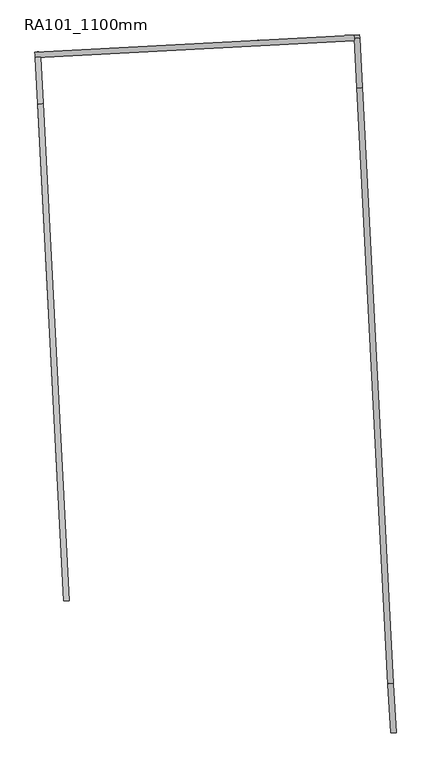
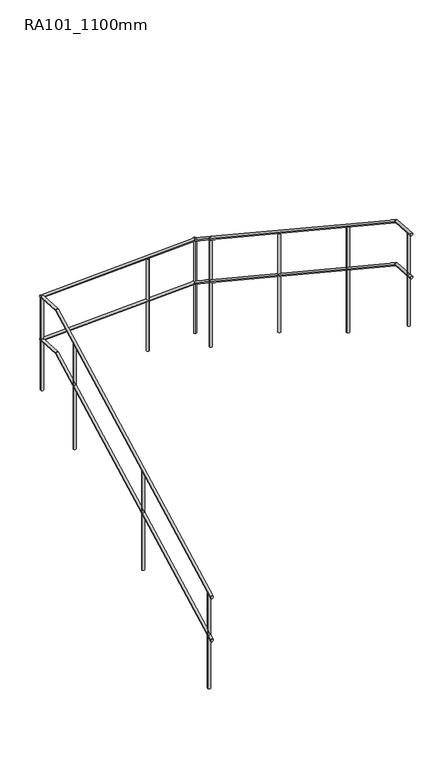
"""IFC4 building model written with IfcOpenShell, lengths in millimetres: railing geometry, RA101_1100mm."""

from ifc_helpers import new_model, si_unit, point, frame, frame_2d, origin, place, context, project, spatial, circle_curve, ellipse_curve, trimmed, segment, composite_curve, outline, extrude, source, transform, mapped, element, save
from ifc_brep_helpers import plane_surface, cylinder_surface, advanced_brep


def ra101_1100mm_54c19647(model_context):
    return source(origin(), model_context, "Body", "SolidModel", [
        advanced_brep(
        [(22896.1789103, 12534.7141331, 457.1248327), (22926.1377964, 12536.2842117, 457.1248327), (22754.6396676, 15235.4437699, 2210.0), (22784.5985536, 15237.0138486, 2210.0), (22741.5052252, 15486.0638601, 2210.0), (22771.4641113, 15487.6339388, 2210.0)],
        [
            (0, 1, ellipse_curve(frame((22911.1583533, 12535.4991724, 457.1248327), z_axis=(0.05233595624294174, -0.998629534754574, 0.0), x_axis=(0.0, 0.0, -0.9999999999999999)), 17.8751673, 15.0)),
            (1, 0, ellipse_curve(frame((22911.1583533, 12535.4991724, 457.1248327), z_axis=(0.05233595624294174, -0.998629534754574, 0.0), x_axis=(0.0, 0.0, -0.9999999999999999)), 17.8751673, 15.0)),
            (0, 2),
            (2, 3, ellipse_curve(frame((22769.6191106, 15236.2288092, 2210.0), z_axis=(0.05018733030882238, -0.9576313096148807, -0.28359038545367066), x_axis=(-0.014841974004015643, 0.28320173468646914, -0.9589455111101144)), 15.6421818, 15.0)),
            (3, 1),
            (3, 2, ellipse_curve(frame((22769.6191106, 15236.2288092, 2210.0), z_axis=(0.05018733030882238, -0.9576313096148807, -0.28359038545367066), x_axis=(-0.014841974004015643, 0.28320173468646914, -0.9589455111101144)), 15.6421818, 15.0)),
            (4, 5, circle_curve(frame((22756.4846683, 15486.8488994, 2210.0), z_axis=(-0.05233595624293797, 0.9986295347545743, 0.0), x_axis=(0.9986295347545743, 0.05233595624293797, 0.0)), 15.0)),
            (5, 4, circle_curve(frame((22756.4846683, 15486.8488994, 2210.0), z_axis=(-0.05233595624293797, 0.9986295347545743, 0.0), x_axis=(0.9986295347545743, 0.05233595624293797, 0.0)), 15.0)),
            (2, 4),
            (5, 3),
        ],
        [
            plane_surface(frame((22911.1583533, 12535.4991724, 475.0), z_axis=(0.05233595624294174, -0.998629534754574, 0.0), x_axis=(0.998629534754574, 0.05233595624294174, 0.0))),
            cylinder_surface(frame((22910.731374, 12543.6464234, 462.4127052), z_axis=(0.04391787398555367, -0.8380029565528062, -0.5438954542495689), x_axis=(0.998629534754574, 0.052335956242941746, 0.0)), 15.0),
            plane_surface(frame((22756.4846683, 15486.8488994, 2225.0), z_axis=(-0.05233595624294184, 0.998629534754574, 0.0), x_axis=(0.998629534754574, 0.05233595624294184, 0.0))),
            cylinder_surface(frame((22769.8512715, 15231.7989162, 2210.0), z_axis=(0.05233595624293797, -0.9986295347545743, 0.0), x_axis=(0.9986295347545743, 0.05233595624293797, 0.0)), 15.0),
        ],
        [
            (0, [[1, 2]]),
            (1, [[-1, 3, 4, 5]]),
            (1, [[-2, -5, 6, -3]]),
            (2, [[7, 8]]),
            (3, [[-4, 9, -8, 10]]),
            (3, [[-6, -10, -7, -9]]),
        ],
    ),
        advanced_brep(
        [(22739.9351465, 15516.0227461, 2210.0), (22741.5052252, 15486.0638601, 2210.0), (24475.8528668, 15606.9983388, 2210.0), (24477.4229455, 15577.0394528, 2210.0)],
        [
            (0, 1, circle_curve(frame((22740.7201859, 15501.0433031, 2210.0), z_axis=(-0.998629534754574, -0.05233595624294185, 0.0), x_axis=(0.05233595624294185, -0.998629534754574, 0.0)), 15.0)),
            (1, 0, circle_curve(frame((22740.7201859, 15501.0433031, 2210.0), z_axis=(-0.998629534754574, -0.05233595624294185, 0.0), x_axis=(0.05233595624294185, -0.998629534754574, 0.0)), 15.0)),
            (2, 3, circle_curve(frame((24476.6379061, 15592.0188958, 2210.0), z_axis=(0.998629534754574, 0.05233595624294185, 0.0), x_axis=(0.05233595624294185, -0.998629534754574, 0.0)), 15.0)),
            (3, 2, circle_curve(frame((24476.6379061, 15592.0188958, 2210.0), z_axis=(0.998629534754574, 0.05233595624294185, 0.0), x_axis=(0.05233595624294185, -0.998629534754574, 0.0)), 15.0)),
            (0, 2),
            (3, 1),
        ],
        [
            plane_surface(frame((22740.7201859, 15501.0433031, 2225.0), z_axis=(-0.9986295347545743, -0.052335956242937944, 0.0), x_axis=(0.052335956242937944, -0.9986295347545743, 0.0))),
            plane_surface(frame((24476.6379061, 15592.0188958, 2225.0), z_axis=(0.9986295347545743, 0.052335956242937104, 0.0), x_axis=(0.052335956242937104, -0.9986295347545743, 0.0))),
            cylinder_surface(frame((22740.7201859, 15501.0433031, 2210.0), z_axis=(-0.998629534754574, -0.05233595624294185, 0.0), x_axis=(0.05233595624294185, -0.998629534754574, 0.0)), 15.0),
        ],
        [
            (0, [[1, 2]]),
            (1, [[3, 4]]),
            (2, [[-1, 5, -4, 6]]),
            (2, [[-2, -6, -3, -5]]),
        ],
    ),
        advanced_brep(
        [(24505.8117528, 15608.5684175, 2210.0), (24475.8528668, 15606.9983388, 2210.0), (24506.8498874, 15588.7596297, 2210.0), (24476.8910014, 15587.189551, 2210.0), (24520.7484348, 15323.5595483, 2382.1248327), (24490.7895487, 15321.9894696, 2382.1248327)],
        [
            (0, 1, circle_curve(frame((24490.8323098, 15607.7833782, 2210.0), z_axis=(-0.052335956242937104, 0.9986295347545743, 0.0), x_axis=(-0.9986295347545743, -0.052335956242937104, 0.0)), 15.0)),
            (1, 0, circle_curve(frame((24490.8323098, 15607.7833782, 2210.0), z_axis=(-0.052335956242937104, 0.9986295347545743, 0.0), x_axis=(-0.9986295347545743, -0.052335956242937104, 0.0)), 15.0)),
            (0, 2),
            (2, 3, ellipse_curve(frame((24491.8704444, 15587.9745903, 2210.0), z_axis=(-0.050187330308819895, 0.9576313096148807, -0.28359038545367116), x_axis=(-0.014841974004020982, 0.2832017346864703, 0.9589455111101142)), 15.6421818, 15.0)),
            (3, 1),
            (3, 2, ellipse_curve(frame((24491.8704444, 15587.9745903, 2210.0), z_axis=(-0.050187330308819895, 0.9576313096148807, -0.28359038545367116), x_axis=(-0.014841974004020982, 0.2832017346864703, 0.9589455111101142)), 15.6421818, 15.0)),
            (4, 5, ellipse_curve(frame((24505.7689917, 15322.774509, 2382.1248327), z_axis=(0.052335956242937104, -0.9986295347545743, 0.0), x_axis=(0.0, 0.0, -1.0)), 17.8751673, 15.0)),
            (5, 4, ellipse_curve(frame((24505.7689917, 15322.774509, 2382.1248327), z_axis=(0.052335956242937104, -0.9986295347545743, 0.0), x_axis=(0.0, 0.0, -1.0)), 17.8751673, 15.0)),
            (2, 4),
            (5, 3),
        ],
        [
            plane_surface(frame((24490.8323098, 15607.7833782, 2225.0), z_axis=(-0.05233595624294184, 0.998629534754574, 0.0), x_axis=(0.998629534754574, 0.05233595624294184, 0.0))),
            cylinder_surface(frame((24490.8323098, 15607.7833782, 2210.0), z_axis=(-0.052335956242937104, 0.9986295347545743, 0.0), x_axis=(-0.9986295347545743, -0.052335956242937104, 0.0)), 15.0),
            plane_surface(frame((24505.7689917, 15322.774509, 2400.0), z_axis=(0.052335956242937104, -0.9986295347545743, 0.0), x_axis=(0.9986295347545743, 0.052335956242937104, 0.0))),
            cylinder_surface(frame((24492.0652629, 15584.2572324, 2212.4127052), z_axis=(-0.04391787398554974, 0.8380029565528057, -0.5438954542495701), x_axis=(-0.9986295347545743, -0.0523359562429371, 0.0)), 15.0),
        ],
        [
            (0, [[1, 2]]),
            (1, [[-1, 3, 4, 5]]),
            (1, [[-2, -5, 6, -3]]),
            (2, [[7, 8]]),
            (3, [[-4, 9, -8, 10]]),
            (3, [[-6, -10, -7, -9]]),
        ],
    ),
        advanced_brep(
        [(24520.7484348, 15323.5595483, 2382.1248327), (24490.7895487, 15321.9894696, 2382.1248327), (24690.5490938, 12083.5699627, 4485.0), (24660.5902078, 12081.999884, 4485.0), (24704.4476412, 11818.3698813, 4485.0), (24674.4887551, 11816.7998026, 4485.0)],
        [
            (0, 1, ellipse_curve(frame((24505.7689917, 15322.774509, 2382.1248327), z_axis=(-0.05233595624294191, 0.998629534754574, 0.0), x_axis=(0.0, 0.0, -1.0)), 17.8751673, 15.0)),
            (1, 0, ellipse_curve(frame((24505.7689917, 15322.774509, 2382.1248327), z_axis=(-0.05233595624294191, 0.998629534754574, 0.0), x_axis=(0.0, 0.0, -1.0)), 17.8751673, 15.0)),
            (0, 2),
            (2, 3, ellipse_curve(frame((24675.5696508, 12082.7849234, 4485.0), z_axis=(-0.05018733030882025, 0.9576313096148807, -0.28359038545367127), x_axis=(0.014841974004007963, -0.28320173468647103, -0.9589455111101143)), 15.6421818, 15.0)),
            (3, 1),
            (3, 2, ellipse_curve(frame((24675.5696508, 12082.7849234, 4485.0), z_axis=(-0.05018733030882025, 0.9576313096148807, -0.28359038545367127), x_axis=(0.014841974004007963, -0.28320173468647103, -0.9589455111101143)), 15.6421818, 15.0)),
            (4, 5, circle_curve(frame((24689.4681982, 11817.584842, 4485.0), z_axis=(0.05233595624293375, -0.9986295347545745, 0.0), x_axis=(-0.9986295347545745, -0.05233595624293375, 0.0)), 15.0)),
            (5, 4, circle_curve(frame((24689.4681982, 11817.584842, 4485.0), z_axis=(0.05233595624293375, -0.9986295347545745, 0.0), x_axis=(-0.9986295347545745, -0.05233595624293375, 0.0)), 15.0)),
            (2, 4),
            (5, 3),
        ],
        [
            plane_surface(frame((24505.7689917, 15322.774509, 2400.0), z_axis=(-0.05233595624294191, 0.998629534754574, 0.0), x_axis=(0.998629534754574, 0.05233595624294191, 0.0))),
            cylinder_surface(frame((24506.1959711, 15314.627258, 2387.4127052), z_axis=(-0.04391787398555378, 0.8380029565528053, -0.5438954542495702), x_axis=(-0.998629534754574, -0.052335956242941926, 0.0)), 15.0),
            plane_surface(frame((24689.4681982, 11817.584842, 4500.0), z_axis=(0.05233595624293375, -0.9986295347545745, 0.0), x_axis=(0.9986295347545745, 0.05233595624293375, 0.0))),
            cylinder_surface(frame((24675.33749, 12087.2148164, 4485.0), z_axis=(-0.05233595624293375, 0.9986295347545745, 0.0), x_axis=(-0.9986295347545745, -0.05233595624293375, 0.0)), 15.0),
        ],
        [
            (0, [[1, 2]]),
            (1, [[-1, 3, 4, 5]]),
            (1, [[-2, -5, 6, -3]]),
            (2, [[7, 8]]),
            (3, [[-4, 9, -8, 10]]),
            (3, [[-6, -10, -7, -9]]),
        ],
    ),
        advanced_brep(
        [(22896.1789103, 12534.7141331, 957.1248327), (22926.1377964, 12536.2842117, 957.1248327), (22754.6396676, 15235.4437699, 2710.0), (22784.5985536, 15237.0138486, 2710.0), (22741.5052252, 15486.0638601, 2710.0), (22771.4641113, 15487.6339388, 2710.0)],
        [
            (0, 1, ellipse_curve(frame((22911.1583533, 12535.4991724, 957.1248327), z_axis=(0.05233595624294174, -0.998629534754574, 0.0), x_axis=(0.0, 0.0, -0.9999999999999999)), 17.8751673, 15.0)),
            (1, 0, ellipse_curve(frame((22911.1583533, 12535.4991724, 957.1248327), z_axis=(0.05233595624294174, -0.998629534754574, 0.0), x_axis=(0.0, 0.0, -0.9999999999999999)), 17.8751673, 15.0)),
            (0, 2),
            (2, 3, ellipse_curve(frame((22769.6191106, 15236.2288092, 2710.0), z_axis=(0.05018733030882238, -0.9576313096148807, -0.28359038545367066), x_axis=(-0.014841974004015643, 0.28320173468646914, -0.9589455111101144)), 15.6421818, 15.0)),
            (3, 1),
            (3, 2, ellipse_curve(frame((22769.6191106, 15236.2288092, 2710.0), z_axis=(0.05018733030882238, -0.9576313096148807, -0.28359038545367066), x_axis=(-0.014841974004015643, 0.28320173468646914, -0.9589455111101144)), 15.6421818, 15.0)),
            (4, 5, circle_curve(frame((22756.4846683, 15486.8488994, 2710.0), z_axis=(-0.05233595624293797, 0.9986295347545743, 0.0), x_axis=(0.9986295347545743, 0.05233595624293797, 0.0)), 15.0)),
            (5, 4, circle_curve(frame((22756.4846683, 15486.8488994, 2710.0), z_axis=(-0.05233595624293797, 0.9986295347545743, 0.0), x_axis=(0.9986295347545743, 0.05233595624293797, 0.0)), 15.0)),
            (2, 4),
            (5, 3),
        ],
        [
            plane_surface(frame((22911.1583533, 12535.4991724, 975.0), z_axis=(0.05233595624294174, -0.998629534754574, 0.0), x_axis=(0.998629534754574, 0.05233595624294174, 0.0))),
            cylinder_surface(frame((22910.731374, 12543.6464234, 962.4127052), z_axis=(0.04391787398555367, -0.8380029565528062, -0.5438954542495689), x_axis=(0.998629534754574, 0.052335956242941746, 0.0)), 15.0),
            plane_surface(frame((22756.4846683, 15486.8488994, 2725.0), z_axis=(-0.05233595624294184, 0.998629534754574, 0.0), x_axis=(0.998629534754574, 0.05233595624294184, 0.0))),
            cylinder_surface(frame((22769.8512715, 15231.7989162, 2710.0), z_axis=(0.05233595624293797, -0.9986295347545743, 0.0), x_axis=(0.9986295347545743, 0.05233595624293797, 0.0)), 15.0),
        ],
        [
            (0, [[1, 2]]),
            (1, [[-1, 3, 4, 5]]),
            (1, [[-2, -5, 6, -3]]),
            (2, [[7, 8]]),
            (3, [[-4, 9, -8, 10]]),
            (3, [[-6, -10, -7, -9]]),
        ],
    ),
        advanced_brep(
        [(22739.9351465, 15516.0227461, 2710.0), (22741.5052252, 15486.0638601, 2710.0), (24475.8528668, 15606.9983388, 2710.0), (24477.4229455, 15577.0394528, 2710.0)],
        [
            (0, 1, circle_curve(frame((22740.7201859, 15501.0433031, 2710.0), z_axis=(-0.998629534754574, -0.05233595624294185, 0.0), x_axis=(0.05233595624294185, -0.998629534754574, 0.0)), 15.0)),
            (1, 0, circle_curve(frame((22740.7201859, 15501.0433031, 2710.0), z_axis=(-0.998629534754574, -0.05233595624294185, 0.0), x_axis=(0.05233595624294185, -0.998629534754574, 0.0)), 15.0)),
            (2, 3, circle_curve(frame((24476.6379061, 15592.0188958, 2710.0), z_axis=(0.998629534754574, 0.05233595624294185, 0.0), x_axis=(0.05233595624294185, -0.998629534754574, 0.0)), 15.0)),
            (3, 2, circle_curve(frame((24476.6379061, 15592.0188958, 2710.0), z_axis=(0.998629534754574, 0.05233595624294185, 0.0), x_axis=(0.05233595624294185, -0.998629534754574, 0.0)), 15.0)),
            (0, 2),
            (3, 1),
        ],
        [
            plane_surface(frame((22740.7201859, 15501.0433031, 2725.0), z_axis=(-0.9986295347545743, -0.052335956242937944, 0.0), x_axis=(0.052335956242937944, -0.9986295347545743, 0.0))),
            plane_surface(frame((24476.6379061, 15592.0188958, 2725.0), z_axis=(0.9986295347545743, 0.052335956242937104, 0.0), x_axis=(0.052335956242937104, -0.9986295347545743, 0.0))),
            cylinder_surface(frame((22740.7201859, 15501.0433031, 2710.0), z_axis=(-0.998629534754574, -0.05233595624294185, 0.0), x_axis=(0.05233595624294185, -0.998629534754574, 0.0)), 15.0),
        ],
        [
            (0, [[1, 2]]),
            (1, [[3, 4]]),
            (2, [[-1, 5, -4, 6]]),
            (2, [[-2, -6, -3, -5]]),
        ],
    ),
        advanced_brep(
        [(24505.8117528, 15608.5684175, 2710.0), (24475.8528668, 15606.9983388, 2710.0), (24506.8498874, 15588.7596297, 2710.0), (24476.8910014, 15587.189551, 2710.0), (24520.7484348, 15323.5595483, 2882.1248327), (24490.7895487, 15321.9894696, 2882.1248327)],
        [
            (0, 1, circle_curve(frame((24490.8323098, 15607.7833782, 2710.0), z_axis=(-0.052335956242937104, 0.9986295347545743, 0.0), x_axis=(-0.9986295347545743, -0.052335956242937104, 0.0)), 15.0)),
            (1, 0, circle_curve(frame((24490.8323098, 15607.7833782, 2710.0), z_axis=(-0.052335956242937104, 0.9986295347545743, 0.0), x_axis=(-0.9986295347545743, -0.052335956242937104, 0.0)), 15.0)),
            (0, 2),
            (2, 3, ellipse_curve(frame((24491.8704444, 15587.9745903, 2710.0), z_axis=(-0.050187330308819895, 0.9576313096148807, -0.28359038545367116), x_axis=(-0.014841974004020982, 0.2832017346864703, 0.9589455111101142)), 15.6421818, 15.0)),
            (3, 1),
            (3, 2, ellipse_curve(frame((24491.8704444, 15587.9745903, 2710.0), z_axis=(-0.050187330308819895, 0.9576313096148807, -0.28359038545367116), x_axis=(-0.014841974004020982, 0.2832017346864703, 0.9589455111101142)), 15.6421818, 15.0)),
            (4, 5, ellipse_curve(frame((24505.7689917, 15322.774509, 2882.1248327), z_axis=(0.052335956242937104, -0.9986295347545743, 0.0), x_axis=(0.0, 0.0, -1.0)), 17.8751673, 15.0)),
            (5, 4, ellipse_curve(frame((24505.7689917, 15322.774509, 2882.1248327), z_axis=(0.052335956242937104, -0.9986295347545743, 0.0), x_axis=(0.0, 0.0, -1.0)), 17.8751673, 15.0)),
            (2, 4),
            (5, 3),
        ],
        [
            plane_surface(frame((24490.8323098, 15607.7833782, 2725.0), z_axis=(-0.05233595624294184, 0.998629534754574, 0.0), x_axis=(0.998629534754574, 0.05233595624294184, 0.0))),
            cylinder_surface(frame((24490.8323098, 15607.7833782, 2710.0), z_axis=(-0.052335956242937104, 0.9986295347545743, 0.0), x_axis=(-0.9986295347545743, -0.052335956242937104, 0.0)), 15.0),
            plane_surface(frame((24505.7689917, 15322.774509, 2900.0), z_axis=(0.052335956242937104, -0.9986295347545743, 0.0), x_axis=(0.9986295347545743, 0.052335956242937104, 0.0))),
            cylinder_surface(frame((24492.0652629, 15584.2572324, 2712.4127052), z_axis=(-0.04391787398554974, 0.8380029565528057, -0.5438954542495701), x_axis=(-0.9986295347545743, -0.0523359562429371, 0.0)), 15.0),
        ],
        [
            (0, [[1, 2]]),
            (1, [[-1, 3, 4, 5]]),
            (1, [[-2, -5, 6, -3]]),
            (2, [[7, 8]]),
            (3, [[-4, 9, -8, 10]]),
            (3, [[-6, -10, -7, -9]]),
        ],
    ),
        advanced_brep(
        [(24520.7484348, 15323.5595483, 2882.1248327), (24490.7895487, 15321.9894696, 2882.1248327), (24690.5490938, 12083.5699627, 4985.0), (24660.5902078, 12081.999884, 4985.0), (24704.4476412, 11818.3698813, 4985.0), (24674.4887551, 11816.7998026, 4985.0)],
        [
            (0, 1, ellipse_curve(frame((24505.7689917, 15322.774509, 2882.1248327), z_axis=(-0.05233595624294191, 0.998629534754574, 0.0), x_axis=(0.0, 0.0, -1.0)), 17.8751673, 15.0)),
            (1, 0, ellipse_curve(frame((24505.7689917, 15322.774509, 2882.1248327), z_axis=(-0.05233595624294191, 0.998629534754574, 0.0), x_axis=(0.0, 0.0, -1.0)), 17.8751673, 15.0)),
            (0, 2),
            (2, 3, ellipse_curve(frame((24675.5696508, 12082.7849234, 4985.0), z_axis=(-0.05018733030882025, 0.9576313096148807, -0.28359038545367127), x_axis=(0.014841974004007963, -0.28320173468647103, -0.9589455111101143)), 15.6421818, 15.0)),
            (3, 1),
            (3, 2, ellipse_curve(frame((24675.5696508, 12082.7849234, 4985.0), z_axis=(-0.05018733030882025, 0.9576313096148807, -0.28359038545367127), x_axis=(0.014841974004007963, -0.28320173468647103, -0.9589455111101143)), 15.6421818, 15.0)),
            (4, 5, circle_curve(frame((24689.4681982, 11817.584842, 4985.0), z_axis=(0.05233595624293375, -0.9986295347545745, 0.0), x_axis=(-0.9986295347545745, -0.05233595624293375, 0.0)), 15.0)),
            (5, 4, circle_curve(frame((24689.4681982, 11817.584842, 4985.0), z_axis=(0.05233595624293375, -0.9986295347545745, 0.0), x_axis=(-0.9986295347545745, -0.05233595624293375, 0.0)), 15.0)),
            (2, 4),
            (5, 3),
        ],
        [
            plane_surface(frame((24505.7689917, 15322.774509, 2900.0), z_axis=(-0.05233595624294191, 0.998629534754574, 0.0), x_axis=(0.998629534754574, 0.05233595624294191, 0.0))),
            cylinder_surface(frame((24506.1959711, 15314.627258, 2887.4127052), z_axis=(-0.04391787398555378, 0.8380029565528053, -0.5438954542495702), x_axis=(-0.998629534754574, -0.052335956242941926, 0.0)), 15.0),
            plane_surface(frame((24689.4681982, 11817.584842, 5000.0), z_axis=(0.05233595624293375, -0.9986295347545745, 0.0), x_axis=(0.9986295347545745, 0.05233595624293375, 0.0))),
            cylinder_surface(frame((24675.33749, 12087.2148164, 4985.0), z_axis=(-0.05233595624293375, 0.9986295347545745, 0.0), x_axis=(-0.9986295347545745, -0.05233595624293375, 0.0)), 15.0),
        ],
        [
            (0, [[1, 2]]),
            (1, [[-1, 3, 4, 5]]),
            (1, [[-2, -5, 6, -3]]),
            (2, [[7, 8]]),
            (3, [[-4, 9, -8, 10]]),
            (3, [[-6, -10, -7, -9]]),
        ],
    ),
        extrude(outline(composite_curve([segment(trimmed(circle_curve(frame_2d((24631.3752867, 12926.0636256)), 15.0), [point((24616.3958437, 12925.2785862))], [point((24646.3547297, 12926.8486649))], False, "CARTESIAN"), True, "CONTINUOUS"), segment(trimmed(circle_curve(frame_2d((24631.3752867, 12926.0636256)), 15.0), [point((24646.3547297, 12926.8486649))], [point((24616.3958437, 12925.2785862))], False, "CARTESIAN"), True, "CONTINUOUS")], self_intersect=False)), frame((0.0, 0.0, 3200.0), z_axis=(0.0, 0.0, 1.0), x_axis=(1.0, 0.0, 0.0)), (0.0, 0.0, 1.0), 1225.5555556),
        extrude(outline(composite_curve([segment(trimmed(circle_curve(frame_2d((24568.5721392, 14124.4190673)), 15.0), [point((24553.5926962, 14123.6340279))], [point((24583.5515823, 14125.2041066))], False, "CARTESIAN"), True, "CONTINUOUS"), segment(trimmed(circle_curve(frame_2d((24568.5721392, 14124.4190673)), 15.0), [point((24583.5515823, 14125.2041066))], [point((24553.5926962, 14123.6340279))], False, "CARTESIAN"), True, "CONTINUOUS")], self_intersect=False)), frame((0.0, 0.0, 2500.0), z_axis=(0.0, 0.0, 1.0), x_axis=(1.0, 0.0, 0.0)), (0.0, 0.0, 1.0), 1147.7777778),
        extrude(outline(composite_curve([segment(trimmed(circle_curve(frame_2d((23954.0550706, 15564.6314899)), 15.0), [point((23954.84011, 15549.6520469))], [point((23953.2700313, 15579.6109329))], False, "CARTESIAN"), True, "CONTINUOUS"), segment(trimmed(circle_curve(frame_2d((23954.0550706, 15564.6314899)), 15.0), [point((23953.2700313, 15579.6109329))], [point((23954.84011, 15549.6520469))], False, "CARTESIAN"), True, "CONTINUOUS")], self_intersect=False)), frame((0.0, 0.0, 1625.0), z_axis=(0.0, 0.0, 1.0), x_axis=(1.0, 0.0, 0.0)), (0.0, 0.0, 1.0), 1070.0),
        extrude(outline(composite_curve([segment(trimmed(circle_curve(frame_2d((22785.5520583, 14932.2100558)), 15.0), [point((22800.5315014, 14932.9950952))], [point((22770.5726153, 14931.4250165))], False, "CARTESIAN"), True, "CONTINUOUS"), segment(trimmed(circle_curve(frame_2d((22785.5520583, 14932.2100558)), 15.0), [point((22770.5726153, 14931.4250165))], [point((22800.5315014, 14932.9950952))], False, "CARTESIAN"), True, "CONTINUOUS")], self_intersect=False)), frame((0.0, 0.0, 1275.0), z_axis=(0.0, 0.0, 1.0), x_axis=(1.0, 0.0, 0.0)), (0.0, 0.0, 1.0), 1225.5555556),
        extrude(outline(composite_curve([segment(trimmed(circle_curve(frame_2d((22848.3552058, 13733.8546141)), 15.0), [point((22863.3346489, 13734.6396534))], [point((22833.3757628, 13733.0695748))], False, "CARTESIAN"), True, "CONTINUOUS"), segment(trimmed(circle_curve(frame_2d((22848.3552058, 13733.8546141)), 15.0), [point((22833.3757628, 13733.0695748))], [point((22863.3346489, 13734.6396534))], False, "CARTESIAN"), True, "CONTINUOUS")], self_intersect=False)), frame((0.0, 0.0, 575.0), z_axis=(0.0, 0.0, 1.0), x_axis=(1.0, 0.0, 0.0)), (0.0, 0.0, 1.0), 1147.7777778),
        extrude(outline(composite_curve([segment(trimmed(circle_curve(frame_2d((24505.7689917, 15322.774509)), 15.0), [point((24490.7895487, 15321.9894696))], [point((24520.7484348, 15323.5595483))], False, "CARTESIAN"), True, "CONTINUOUS"), segment(trimmed(circle_curve(frame_2d((24505.7689917, 15322.774509)), 15.0), [point((24520.7484348, 15323.5595483))], [point((24490.7895487, 15321.9894696))], False, "CARTESIAN"), True, "CONTINUOUS")], self_intersect=False)), frame((0.0, 0.0, 1625.0), z_axis=(0.0, 0.0, 1.0), x_axis=(1.0, 0.0, 0.0)), (0.0, 0.0, 1.0), 1245.0),
        extrude(outline(composite_curve([segment(trimmed(circle_curve(frame_2d((24491.6173492, 15592.8039352)), 15.0), [point((24492.4023885, 15577.8244921))], [point((24490.8323098, 15607.7833782))], False, "CARTESIAN"), True, "CONTINUOUS"), segment(trimmed(circle_curve(frame_2d((24491.6173492, 15592.8039352)), 15.0), [point((24490.8323098, 15607.7833782))], [point((24492.4023885, 15577.8244921))], False, "CARTESIAN"), True, "CONTINUOUS")], self_intersect=False)), frame((0.0, 0.0, 1625.0), z_axis=(0.0, 0.0, 1.0), x_axis=(1.0, 0.0, 0.0)), (0.0, 0.0, 1.0), 1070.0),
        extrude(outline(composite_curve([segment(trimmed(circle_curve(frame_2d((22755.6996289, 15501.8283424)), 15.0), [point((22770.6790719, 15502.6133818))], [point((22740.7201859, 15501.0433031))], False, "CARTESIAN"), True, "CONTINUOUS"), segment(trimmed(circle_curve(frame_2d((22755.6996289, 15501.8283424)), 15.0), [point((22740.7201859, 15501.0433031))], [point((22770.6790719, 15502.6133818))], False, "CARTESIAN"), True, "CONTINUOUS")], self_intersect=False)), frame((0.0, 0.0, 1625.0), z_axis=(0.0, 0.0, 1.0), x_axis=(1.0, 0.0, 0.0)), (0.0, 0.0, 1.0), 1070.0),
        extrude(outline(composite_curve([segment(trimmed(circle_curve(frame_2d((24686.8514003, 11867.5163187)), 15.0), [point((24671.8719573, 11866.7312794))], [point((24701.8308434, 11868.3013581))], False, "CARTESIAN"), True, "CONTINUOUS"), segment(trimmed(circle_curve(frame_2d((24686.8514003, 11867.5163187)), 15.0), [point((24701.8308434, 11868.3013581))], [point((24671.8719573, 11866.7312794))], False, "CARTESIAN"), True, "CONTINUOUS")], self_intersect=False)), frame((0.0, 0.0, 3900.0), z_axis=(0.0, 0.0, 1.0), x_axis=(1.0, 0.0, 0.0)), (0.0, 0.0, 1.0), 1070.0),
        extrude(outline(composite_curve([segment(trimmed(circle_curve(frame_2d((22908.5415555, 12585.4306491)), 15.0), [point((22923.5209985, 12586.2156885))], [point((22893.5621125, 12584.6456098))], False, "CARTESIAN"), True, "CONTINUOUS"), segment(trimmed(circle_curve(frame_2d((22908.5415555, 12585.4306491)), 15.0), [point((22893.5621125, 12584.6456098))], [point((22923.5209985, 12586.2156885))], False, "CARTESIAN"), True, "CONTINUOUS")], self_intersect=False)), frame((0.0, 0.0, -125.0), z_axis=(0.0, 0.0, 1.0), x_axis=(1.0, 0.0, 0.0)), (0.0, 0.0, 1.0), 1102.4074074),
    ])


if __name__ == "__main__":
    model = new_model("IFC4")
    model_context = context("Model", 3, world=origin())
    ifc_project = project(units=[si_unit("LENGTHUNIT", "METRE", prefix="MILLI")], contexts=[model_context])
    site = spatial("IfcSite", under=ifc_project)
    building = spatial("IfcBuilding", under=site)
    placement = place(None, origin())
    ra101_1100mm_shape = ra101_1100mm_54c19647(model_context)
    element("IfcRailing", 1, ObjectType="RA101_1100mm", at=placement, inside=building, context=model_context, shape_type="MappedRepresentation", body=[
        mapped(ra101_1100mm_shape, transform((0.0, 0.0, 0.0), x_axis=(1.0, 0.0, 0.0), y_axis=(0.0, 1.0, 0.0), z_axis=(0.0, 0.0, 1.0))),
    ])
    save(model, "model.ifc")
